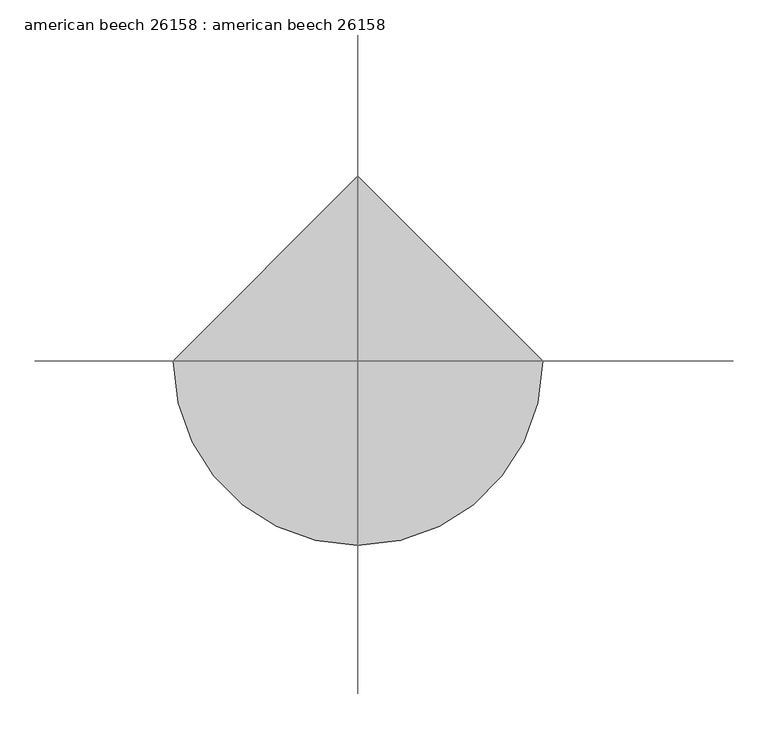
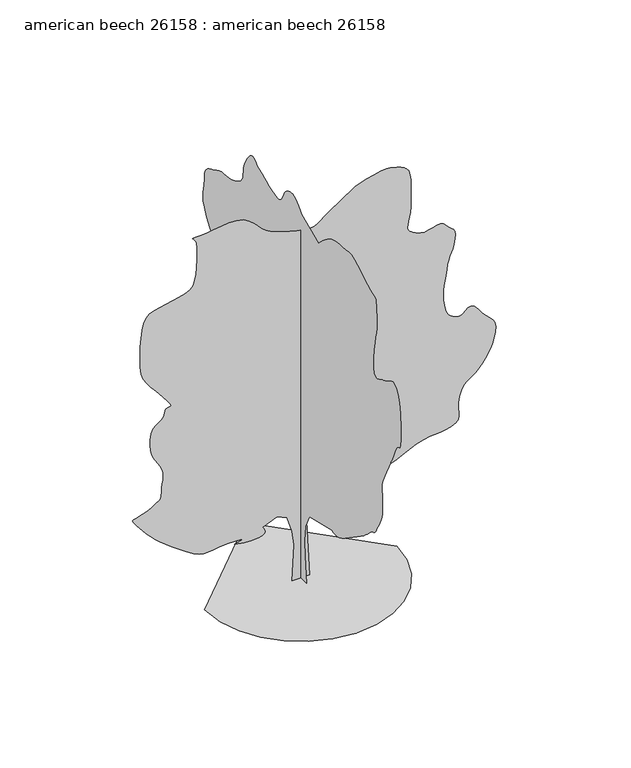
"""IFC4 building model written with IfcOpenShell, lengths in millimetres: proxy geometry, american beech 26158 : american beech 26158."""

from ifc_helpers import new_model, si_unit, origin, place, context, project, spatial, triangles, source, transform, mapped, element, save


def american_beech_26158_american_beech_26158_b3c041c8(model_context):
    return source(origin(), model_context, "Body", "Tessellation", [
        triangles([(0.0009889, 136.856581, 0.0), (0.0009889, -149.8547884, 0.0), (0.0009889, -111.6264895, 420.510052), (0.0009889, -102.0697236, 659.4353302), (0.0009889, -121.1832463, 898.3606447), (0.0009889, -235.8678885, 1118.172373), (0.0009889, -818.8458761, 1261.5275036), (0.0009889, -849.9431059, 1249.7139805), (0.0009889, -883.2933231, 1240.7427258), (0.0009889, -921.1596891, 1237.4533916), (0.0009889, -965.7976622, 1242.6934788), (0.0009889, -1019.4603024, 1259.3000233), (0.0009889, -1084.4081549, 1290.1152935), (0.0009889, -1162.8992941, 1337.984174), (0.0009889, -1478.2811337, 1557.7959023), (0.0009889, -1522.8632961, 1589.1420994), (0.0009889, -1566.942437, 1618.9819931), (0.0009889, -1611.1893002, 1649.3249084), (0.0009889, -1656.2718681, 1682.1772636), (0.0009889, -1702.8579781, 1719.5406807), (0.0009889, -1751.6183739, 1763.4243393), (0.0009889, -1803.2210381, 1815.834803), (0.0009889, -1847.9404015, 1858.0191467), (0.0009889, -1878.9512993, 1877.1351311), (0.0009889, -1901.2702858, 1884.0440117), (0.0009889, -1919.9112991, 1889.616782), (0.0009889, -1939.8884228, 1904.7196392), (0.0009889, -1966.2180656, 1940.2161644), (0.0009889, -2003.916782, 2006.9774963), (0.0009889, -2044.9607883, 2083.2080177), (0.0009889, -2078.313549, 2145.2324295), (0.0009889, -2104.4754696, 2201.0692829), (0.0009889, -2123.9521877, 2258.7475937), (0.0009889, -2137.244109, 2326.2862038), (0.0009889, -2144.8488773, 2411.7141289), (0.0009889, -2147.2746014, 2523.0550072), (0.0009889, -2142.5373905, 2624.8889076), (0.0009889, -2132.7863869, 2688.2873634), (0.0009889, -2124.7040314, 2730.9338882), (0.0009889, -2124.9835201, 2770.583503), (0.0009889, -2140.3072941, 2824.9394875), (0.0009889, -2177.3659332, 2911.7568626), (0.0009889, -2242.84464, 3048.6883301), (0.0009889, -2308.7119858, 3181.9621719), (0.0009889, -2348.5011269, 3259.3812836), (0.0009889, -2371.2366577, 3301.215358), (0.0009889, -2385.9484051, 3327.6567673), (0.0009889, -2401.6632889, 3358.9496246), (0.0009889, -2427.4088104, 3415.3121727), (0.0009889, -2472.2118896, 3516.9885246), (0.0009889, -2522.8114174, 3609.6476944), (0.0009889, -2561.0332123, 3645.1568642), (0.0009889, -2588.5669968, 3652.9040657), (0.0009889, -2607.0580193, 3662.3273277), (0.0009889, -2618.2087921, 3702.8402618), (0.0009889, -2623.669796, 3803.856189), (0.0009889, -2625.117382, 3994.8390083), (0.0009889, -2615.3639076, 4210.713913), (0.0009889, -2589.2271309, 4371.4450905), (0.0009889, -2551.406765, 4483.8402649), (0.0009889, -2506.5400269, 4554.7824463), (0.0009889, -2459.3391289, 4591.1043571), (0.0009889, -2414.4802391, 4599.6895889), (0.0009889, -2376.641851, 4587.3705734), (0.0009889, -2343.8477772, 4566.9491455), (0.0009889, -2310.8862717, 4546.8576393), (0.0009889, -2277.5893215, 4527.4521378), (0.0009889, -2243.7921112, 4509.0116936), (0.0009889, -2209.3243023, 4491.9426773), (0.0009889, -2174.0232594, 4476.5250137), (0.0009889, -2137.7164639, 4463.1392029), (0.0009889, -2096.4236355, 4443.6572525), (0.0009889, -2049.6139927, 4418.4858238), (0.0009889, -2002.3013283, 4400.6805153), (0.0009889, -1959.504958, 4403.2713455), (0.0009889, -1926.2359131, 4439.313913), (0.0009889, -1907.5110386, 4521.8132378), (0.0009889, -1908.3467434, 4663.8246277), (0.0009889, -1923.6450829, 4819.4253044), (0.0009889, -1942.954224, 4940.7356323), (0.0009889, -1963.266647, 5037.9669067), (0.0009889, -1981.572361, 5121.3298416), (0.0009889, -1994.8642822, 5201.0354416), (0.0009889, -2000.1296585, 5287.2429703), (0.0009889, -1994.3614059, 5390.1634323), (0.0009889, -1986.3653824, 5488.9190323), (0.0009889, -1983.048143, 5559.911792), (0.0009889, -1978.5625156, 5609.3407516), (0.0009889, -1967.0562412, 5643.3764648), (0.0009889, -1942.6748806, 5668.2429703), (0.0009889, -1899.5709709, 5690.0869858), (0.0009889, -1831.8926891, 5715.1063889), (0.0009889, -1748.4408062, 5751.9616974), (0.0009889, -1662.820015, 5800.5261749), (0.0009889, -1576.3582867, 5853.7903656), (0.0009889, -1490.4020508, 5904.6919098), (0.0009889, -1406.2848015, 5946.2207703), (0.0009889, -1325.3426491, 5971.3924896), (0.0009889, -1248.913884, 5973.1447083), (0.0009889, -1174.2403896, 5963.3406555), (0.0009889, -1098.5636135, 5956.711409), (0.0009889, -1023.222064, 5950.5641098), (0.0009889, -949.5518515, 5942.2588028), (0.0009889, -878.8914843, 5929.1264648), (0.0009889, -812.5771454, 5908.4509827), (0.0009889, -751.9472706, 5877.5644958), (0.0009889, -697.9494038, 5841.2678741), (0.0009889, -649.9687569, 5805.9618896), (0.0009889, -607.0045916, 5771.4942261), (0.0009889, -568.0511189, 5737.7119858), (0.0009889, -532.1075644, 5704.4128555), (0.0009889, -498.1706097, 5671.4433563), (0.0009889, -465.2369368, 5638.6523346), (0.0009889, -16.056217, 5829.7871796), (0.0009889, 22.8405617, 5872.4339951), (0.0009889, 61.6537222, 5913.023378), (0.0009889, 100.2998553, 5949.3961578), (0.0009889, 138.6950317, 5979.5204819), (0.0009889, 176.7559443, 6001.2883392), (0.0009889, 214.3990318, 6012.5911377), (0.0009889, 251.5404602, 6011.3720261), (0.0009889, 287.2056524, 6002.4312927), (0.0009889, 320.3628219, 5991.305809), (0.0009889, 350.8454089, 5977.0055191), (0.0009889, 378.4856913, 5958.5397858), (0.0009889, 403.1160919, 5934.892392), (0.0009889, 424.5689612, 5905.047702), (0.0009889, 442.6817001, 5868.0144974), (0.0009889, 459.9562634, 5826.9425858), (0.0009889, 480.2407084, 5787.547316), (0.0009889, 505.3740581, 5752.6727005), (0.0009889, 537.1926464, 5725.138916), (0.0009889, 577.5380399, 5707.7911377), (0.0009889, 628.2491524, 5703.5239563), (0.0009889, 691.1650068, 5715.1063889), (0.0009889, 759.6790661, 5736.9754028), (0.0009889, 826.1890326, 5761.3593796), (0.0009889, 891.0251186, 5787.8263687), (0.0009889, 954.5251671, 5815.9694183), (0.0009889, 1017.0218611, 5845.3577408), (0.0009889, 1078.8506453, 5875.5832214), (0.0009889, 1140.3440575, 5906.2412338), (0.0009889, 1169.0715191, 5932.3524307), (0.0009889, 1198.1316639, 5955.3649796), (0.0009889, 1227.8624073, 5972.2052307), (0.0009889, 1258.5938164, 5979.7489563), (0.0009889, 1290.6664227, 5974.9230881), (0.0009889, 1324.4078224, 5954.6539764), (0.0009889, 1360.1557858, 5915.7918137), (0.0009889, 1395.1799561, 5868.217392), (0.0009889, 1426.1908539, 5822.9544571), (0.0009889, 1452.6880737, 5778.8856354), (0.0009889, 1474.1715008, 5734.7912338), (0.0009889, 1490.1379681, 5689.5538788), (0.0009889, 1500.0845993, 5641.9538773), (0.0009889, 1503.510989, 5590.8494385), (0.0009889, 1507.2168674, 5539.3380478), (0.0009889, 1519.1142517, 5491.1793594), (0.0009889, 1540.3740005, 5446.1704788), (0.0009889, 1572.1672634, 5404.1846695), (0.0009889, 1615.6596668, 5365.0428726), (0.0009889, 1672.0274471, 5328.5689362), (0.0009889, 1742.4363762, 5294.5832199), (0.0009889, 1817.5288857, 5269.1836075), (0.0009889, 1887.9378147, 5255.1373718), (0.0009889, 1954.8363476, 5247.4407486), (0.0009889, 2019.3956337, 5241.0911362), (0.0009889, 2082.7839157, 5231.0580276), (0.0009889, 2146.1721977, 5212.3382401), (0.0009889, 2210.7313385, 5179.9024292), (0.0009889, 2276.3498623, 5145.3580261), (0.0009889, 2340.1267834, 5118.8404587), (0.0009889, 2399.0573433, 5093.1356323), (0.0009889, 2450.1315514, 5061.106192), (0.0009889, 2490.3372368, 5015.5136261), (0.0009889, 2516.667025, 4949.193837), (0.0009889, 2526.1132507, 4854.9597633), (0.0009889, 2532.46577, 4758.008123), (0.0009889, 2546.5044479, 4681.9348595), (0.0009889, 2560.7285797, 4617.2411339), (0.0009889, 2567.5865913, 4554.3760757), (0.0009889, 2559.5600464, 4483.8402649), (0.0009889, 2529.1232414, 4396.0578323), (0.0009889, 2468.7702393, 4281.5543564), (0.0009889, 2394.0992157, 4166.6192207), (0.0009889, 2326.6139454, 4078.2525215), (0.0009889, 2267.6553349, 4007.9707649), (0.0009889, 2218.5596397, 3947.1884285), (0.0009889, 2180.6679119, 3887.4223091), (0.0009889, 2155.3111748, 3820.1377533), (0.0009889, 2143.8328056, 3736.8001076), (0.0009889, 2149.4334812, 3646.0204742), (0.0009889, 2171.0820145, 3561.7686401), (0.0009889, 2203.7667927, 3483.5112076), (0.0009889, 2242.4687908, 3410.790937), (0.0009889, 2282.1714546, 3343.1000107), (0.0009889, 2317.8662235, 3279.9047401), (0.0009889, 2344.5311657, 3220.7225967), (0.0009889, 2370.3577869, 3180.6921913), (0.0009889, 2402.5396889, 3164.8934464), (0.0009889, 2434.5538685, 3157.7813805), (0.0009889, 2459.8827003, 3143.8113029), (0.0009889, 2472.0037628, 3107.4638123), (0.0009889, 2464.3963783, 3033.1433487), (0.0009889, 2430.5432121, 2905.3305107), (0.0009889, 2383.9011463, 2761.3378464), (0.0009889, 2340.6017544, 2643.9136185), (0.0009889, 2298.1379219, 2545.7425758), (0.0009889, 2254.0028252, 2459.415287), (0.0009889, 2205.6894951, 2377.6095245), (0.0009889, 2150.6857304, 2292.9614937), (0.0009889, 2086.4897942, 2198.1177189), (0.0009889, 2022.098085, 2102.5196297), (0.0009889, 1968.0723129, 2019.6267242), (0.0009889, 1924.2446102, 1948.102747), (0.0009889, 1890.4447838, 1886.6067913), (0.0009889, 1866.5103436, 1833.8078339), (0.0009889, 1852.2735672, 1788.3620613), (0.0009889, 1847.564407, 1748.9361248), (0.0009889, 1851.5776794, 1721.8800728), (0.0009889, 1860.940044, 1709.2029396), (0.0009889, 1871.6386642, 1703.0459026), (0.0009889, 1879.6624477, 1695.5504299), (0.0009889, 1881.0010288, 1678.8600243), (0.0009889, 1871.6386642, 1645.1186245), (0.0009889, 1847.564407, 1586.4675533), (0.0009889, 1827.5314728, 1524.5828133), (0.0009889, 1825.3850922, 1482.2587978), (0.0009889, 1829.7590984, 1453.3104195), (0.0009889, 1829.2865982, 1431.547649), (0.0009889, 1812.5961926, 1410.7907764), (0.0009889, 1768.3214241, 1384.8497726), (0.0009889, 1685.0958355, 1347.5421661), (0.0009889, 1594.399918, 1309.4244347), (0.0009889, 1528.281134, 1282.5080544), (0.0009889, 1476.2059696, 1262.7823689), (0.0009889, 1427.6412014, 1246.2316349), (0.0009889, 1372.05317, 1228.8453415), (0.0009889, 1298.9138844, 1206.6102161), (0.0009889, 1197.6871416, 1175.5154572), (0.0009889, 1096.069289, 1145.7009253), (0.0009889, 1022.5387482, 1127.7557997), (0.0009889, 967.7331545, 1118.3400227), (0.0009889, 922.2874546, 1114.10329), (0.0009889, 876.8442255, 1111.7080873), (0.0009889, 822.0360884, 1107.806654), (0.0009889, 748.5055475, 1099.0588594), (0.0009889, 662.4935011, 1085.0990284), (0.0009889, 576.4788749, 1068.1292793), (0.0009889, 490.4667558, 1048.6551046), (0.0009889, 404.4521296, 1027.1717503), (0.0009889, 318.4400468, 1004.1847086), (0.0009889, 232.4266923, 980.1943851), (0.0009889, 146.4133378, 955.7037289), (136.1842383, 0.0003154, 0.014068), (-131.4120823, 0.0003154, 0.014068), (-102.7410489, 0.0002819, 563.8778998), (-131.4120823, 0.0002692, 793.2477293), (-207.8684348, 0.0002549, 1032.1729712), (-360.7819027, 0.0002501, 1108.6296415), (-580.5936673, 0.0002549, 1013.0594576), (-562.704425, 0.0002564, 988.5662579), (-548.0765751, 0.000258, 964.5784779), (-539.9688578, 0.0002596, 941.5914362), (-541.6401947, 0.0002612, 920.1080818), (-556.3518694, 0.0002628, 900.6313637), (-587.3627672, 0.0002628, 883.6641581), (-637.9342443, 0.0002644, 869.704327), (-697.421093, 0.0002644, 860.4815615), (-753.4001616, 0.0002644, 856.775683), (-806.4506298, 0.0002644, 857.667271), (-857.1617786, 0.0002644, 862.2366869), (-906.117802, 0.0002644, 869.5645826), (-953.9028214, 0.0002628, 878.731465), (-1001.1011759, 0.0002628, 888.8178406), (-953.2881786, 0.0002628, 900.9945683), (-913.501581, 0.0002612, 912.5008427), (-889.7601522, 0.0002612, 922.6710068), (-890.0954515, 0.0002596, 930.8345346), (-922.5287189, 0.0002596, 936.3235165), (-995.0838833, 0.0002596, 938.4698244), (-1115.7848007, 0.0002596, 936.6028599), (-1242.9524746, 0.0002612, 927.8271601), (-1337.3542706, 0.0002612, 914.3677345), (-1410.6891838, 0.0002612, 903.2500992), (-1474.6617325, 0.0002612, 901.4949738), (-1540.9759987, 0.0002612, 916.12286), (-1621.3340298, 0.0002596, 954.1568756), (-1727.4351116, 0.0002549, 1022.614979), (-1845.0726986, 0.0002501, 1105.8432564), (-1952.34711, 0.0002453, 1184.0549795), (-2049.4209812, 0.0002405, 1258.0858532), (-2136.46436, 0.0002373, 1328.7765965), (-2213.6472942, 0.0002326, 1396.9554291), (-2281.1300938, 0.0002278, 1463.4653229), (-2339.0852772, 0.0002246, 1529.1396572), (-2391.8031349, 0.0002214, 1592.6651402), (-2441.3431343, 0.0002166, 1651.1791557), (-2484.5309052, 0.0002134, 1703.170459), (-2518.1884438, 0.0002118, 1747.1378334), (-2539.1409439, 0.0002103, 1781.577737), (-2544.218541, 0.0002087, 1804.9838665), (-2530.2254997, 0.0002071, 1815.8500637), (-2498.742247, 0.0002071, 1822.7308937), (-2456.2227493, 0.0002071, 1834.628278), (-2406.8475655, 0.0002055, 1850.7065117), (-2354.8003063, 0.0002039, 1870.1272739), (-2304.2568798, 0.0002023, 1892.0551506), (-2259.3978447, 0.0002023, 1915.6542915), (-2224.401725, 0.0002007, 1940.091608), (-2196.9849392, 0.0001991, 1958.6464348), (-2172.4078056, 0.0001991, 1969.1798035), (-2151.1759621, 0.0001975, 1977.7066086), (-2133.7896687, 0.0001975, 1990.2439247), (-2120.7518017, 0.0001959, 2012.8144947), (-2112.5602959, 0.0001927, 2051.4326317), (-2109.7180275, 0.0001895, 2112.118317), (-2105.7607109, 0.0001864, 2181.0514641), (-2096.7894562, 0.0001816, 2242.2935108), (-2087.1476028, 0.0001784, 2298.6891964), (-2081.1861935, 0.0001752, 2353.0781731), (-2083.2487129, 0.000172, 2408.3028545), (-2097.6809715, 0.0001688, 2467.2028931), (-2128.8315411, 0.0001641, 2532.6259346), (-2168.3971493, 0.0001609, 2596.7202782), (-2204.2849297, 0.0001577, 2653.2860115), (-2235.1560104, 0.0001545, 2707.6675758), (-2259.6771881, 0.0001513, 2765.2239464), (-2276.5047947, 0.0001465, 2831.3149704), (-2284.3076614, 0.0001418, 2911.2740433), (-2281.7447365, 0.000137, 3010.4865921), (-2264.5514545, 0.0001306, 3102.7902603), (-2233.1494469, 0.0001274, 3164.9948936), (-2193.2231049, 0.0001242, 3206.8286774), (-2150.4520237, 0.0001226, 3237.9439293), (-2110.525827, 0.0001211, 3268.0682533), (-2079.123674, 0.0001179, 3306.8795471), (-2061.9330082, 0.0001147, 3364.0804161), (-2043.9599773, 0.0001131, 3413.0262657), (-2014.1200836, 0.0001115, 3431.3396828), (-1983.9422745, 0.0001115, 3435.3019409), (-1964.9684326, 0.0001099, 3441.0931572), (-1968.7301216, 0.0001099, 3464.9437363), (-2006.7641373, 0.0001051, 3523.0843735), (-2090.6020432, 9.88e-05, 3631.6948952), (-2191.4121689, 9.24e-05, 3753.7165169), (-2273.3296978, 8.6e-05, 3849.6778107), (-2337.3582024, 8.12e-05, 3932.1009773), (-2384.5031445, 7.65e-05, 4013.5079269), (-2415.7654804, 7.17e-05, 4106.47202), (-2432.1484921, 6.37e-05, 4223.4898773), (-2434.6554611, 5.42e-05, 4377.1345688), (-2429.5297565, 4.46e-05, 4541.5998207), (-2420.5585018, 3.66e-05, 4683.0016548), (-2405.0643894, 3.03e-05, 4801.6705742), (-2380.3781055, 2.39e-05, 4897.9365005), (-2343.822488, 1.91e-05, 4972.1558075), (-2292.720084, 1.59e-05, 5024.6066757), (-2224.401725, 1.43e-05, 5055.6710587), (-2138.4149677, 1.27e-05, 5074.7972168), (-2040.8941761, 1.27e-05, 5092.7292618), (-1939.0274288, 1.11e-05, 5111.8554199), (-1840.0028046, 9.6e-06, 5134.487178), (-1751.0088181, 8e-06, 5162.9604401), (-1679.2334026, 6.4e-06, 5199.612854), (-1631.8649277, 3.2e-06, 5246.8314835), (-1604.1128426, -1.6e-06, 5316.4272354), (-1585.3905842, -6.4e-06, 5411.6010773), (-1574.1890877, -1.27e-05, 5521.6594757), (-1569.0075726, -2.07e-05, 5635.9088974), (-1568.336974, -2.71e-05, 5743.6302292), (-1570.6788368, -3.19e-05, 5834.1305191), (-1574.524387, -3.5e-05, 5896.690654), (-1585.918895, -3.82e-05, 5936.1626633), (-1606.0102558, -3.98e-05, 5965.4230865), (-1625.9315689, -4.14e-05, 5985.9718323), (-1636.825526, -4.14e-05, 5999.3576431), (-1629.8329296, -4.3e-05, 6007.0286865), (-1596.0890591, -4.3e-05, 6010.559285), (-1526.7393677, -4.3e-05, 6011.3976059), (-1428.7715103, -4.3e-05, 6017.8233765), (-1318.7690678, -4.46e-05, 6032.4538788), (-1202.2439129, -4.46e-05, 6048.2529144), (-1084.7180197, -4.46e-05, 6058.184285), (-971.7057318, -4.46e-05, 6055.263533), (-868.7238636, -4.46e-05, 6032.4538788), (-781.2893749, -4.14e-05, 5982.7208679), (-714.8937183, -3.66e-05, 5922.6245361), (-665.5465851, -3.34e-05, 5871.6974121), (-624.5610781, -3.19e-05, 5827.4756927), (-583.2403444, -2.87e-05, 5787.445578), (-532.8924365, -2.71e-05, 5749.0915237), (-464.8228995, -2.39e-05, 5709.8735687), (-370.3373878, -2.23e-05, 5667.3284912), (-260.8632923, -1.91e-05, 5627.3745346), (-155.7366604, -1.75e-05, 5596.9449966), (-58.1322665, -1.59e-05, 5575.0504028), (28.7726351, -1.59e-05, 5560.6739548), (101.8020074, -1.59e-05, 5552.8255966), (157.7788323, -1.43e-05, 5550.4629501), (193.5270681, -1.59e-05, 5552.6477005), (219.2725352, -1.59e-05, 5560.6233765), (247.3583572, -1.59e-05, 5575.4311935), (277.7847885, -1.75e-05, 5595.7770447), (310.5508118, -1.91e-05, 5620.2877579), (345.6587342, -2.07e-05, 5647.6692261), (383.1059761, -2.23e-05, 5676.5232788), (422.8950809, -2.39e-05, 5705.555809), (805.1781057, -3.98e-05, 5963.5947098), (830.3647951, -3.98e-05, 5972.992392), (896.679134, -4.14e-05, 5996.5892075), (990.2426817, -4.3e-05, 6027.5518524), (1097.1817938, -4.62e-05, 6058.9970261), (1203.6180296, -4.62e-05, 6084.1175858), (1295.67789, -4.78e-05, 6096.0046509), (1359.4853325, -4.78e-05, 6087.8516602), (1407.4912685, -4.62e-05, 6070.6556168), (1459.1777939, -4.46e-05, 6056.8128571), (1511.1996185, -4.46e-05, 6041.4457718), (1560.2089817, -4.3e-05, 6019.7540726), (1602.8682964, -4.14e-05, 5986.835733), (1635.8299473, -3.82e-05, 5937.8898834), (1655.7537312, -3.34e-05, 5868.0394958), (1665.3091072, -2.87e-05, 5789.7820633), (1670.1859898, -2.55e-05, 5717.2399796), (1671.5500053, -2.07e-05, 5647.8471222), (1670.5746288, -1.75e-05, 5579.1396881), (1668.4282482, -1.27e-05, 5508.6038773), (1666.2844837, -8e-06, 5433.699147), (1665.3091072, -3.2e-06, 5351.9622757), (1660.2367424, 1.6e-06, 5270.5806152), (1648.1463467, 6.4e-06, 5198.4187408), (1633.7114719, 9.6e-06, 5135.2743393), (1621.6186054, 1.27e-05, 5081.0200928), (1616.5487114, 1.59e-05, 5035.4269455), (1623.1807194, 1.75e-05, 4998.368161), (1646.1955936, 1.91e-05, 4969.6664246), (1678.4054008, 2.07e-05, 4946.8317719), (1709.6119263, 2.23e-05, 4927.324823), (1739.9826015, 2.23e-05, 4910.992099), (1769.6829689, 2.39e-05, 4897.6824463), (1798.8852562, 2.39e-05, 4887.1923889), (1827.7499187, 2.55e-05, 4879.3946091), (1856.4493298, 2.55e-05, 4874.0862122), (1893.0609032, 2.55e-05, 4877.1087021), (1942.2125542, 2.39e-05, 4889.9864044), (1998.8851124, 2.39e-05, 4906.1918106), (2058.0671104, 2.23e-05, 4919.2474091), (2114.7396687, 2.23e-05, 4922.5745316), (2163.8911743, 2.39e-05, 4909.6968292), (2200.5028931, 2.55e-05, 4874.0862122), (2230.4850746, 2.71e-05, 4834.208123), (2261.3003448, 2.87e-05, 4807.6649757), (2290.2766285, 3.03e-05, 4786.8368866), (2314.7419956, 3.19e-05, 4763.9769447), (2332.0165226, 3.34e-05, 4731.4396866), (2339.4282795, 3.66e-05, 4681.5031998), (2334.3025749, 4.14e-05, 4606.4970222), (2319.8956055, 4.62e-05, 4526.9440292), (2302.1485783, 4.94e-05, 4463.951944), (2282.3925167, 5.26e-05, 4410.6627548), (2261.9683273, 5.57e-05, 4360.1928703), (2242.2147366, 5.89e-05, 4305.7098587), (2224.4652386, 6.37e-05, 4240.3809975), (2210.0608852, 6.85e-05, 4157.3229858), (2196.9087811, 7.33e-05, 4068.4481781), (2183.2562714, 7.8e-05, 3988.0827347), (2170.9397266, 8.28e-05, 3913.0762665), (2161.8007496, 8.76e-05, 3840.2289688), (2157.6783268, 9.08e-05, 3766.3913246), (2160.4088287, 9.56e-05, 3688.3876556), (2171.831242, 0.0001003, 3603.0181572), (2189.9719952, 0.0001051, 3525.0147789), (2211.6203831, 0.0001083, 3468.2711494), (2236.7791672, 0.0001115, 3428.240744), (2265.4506729, 0.0001131, 3400.402327), (2297.6324295, 0.0001147, 3380.2602425), (2333.3271984, 0.0001147, 3363.2673843), (2372.5296021, 0.0001163, 3344.9795471), (2412.5675652, 0.0001163, 3342.4901642), (2451.7724396, 0.0001147, 3366.0869797), (2491.642971, 0.0001131, 3400.8848557), (2533.6901138, 0.0001115, 3432.0253967), (2579.4227875, 0.0001099, 3444.5728867), (2630.3246223, 0.0001115, 3423.7195084), (2687.906282, 0.0001163, 3354.5298363), (2749.8568611, 0.0001211, 3269.9730789), (2810.1313797, 0.0001242, 3206.9557045), (2864.6905495, 0.0001274, 3156.6637161), (2909.5976921, 0.0001306, 3110.2325386), (2940.7635223, 0.0001338, 3058.7720169), (2954.2254913, 0.000137, 2993.4178665), (2945.9451828, 0.0001434, 2905.3557999), (2924.1520363, 0.0001481, 2810.6139084), (2899.209082, 0.0001529, 2729.079641), (2870.2277115, 0.0001577, 2657.6040619), (2836.3948929, 0.0001609, 2592.9612053), (2796.8723053, 0.0001641, 2531.9858574), (2750.8474983, 0.0001688, 2471.5235596), (2697.4568619, 0.000172, 2408.3842449), (2642.4404526, 0.0001752, 2354.2186558), (2591.9196991, 0.0001784, 2316.7713776), (2545.7425758, 0.00018, 2287.0127289), (2503.7637428, 0.0001816, 2255.9181152), (2465.7858284, 0.0001832, 2214.4575645), (2431.6531734, 0.000188, 2153.606773), (2401.2011078, 0.0001927, 2064.3332977), (2384.7901909, 0.0001991, 1965.7532684), (2385.7654221, 0.0002039, 1881.8849865), (2393.4261463, 0.0002071, 1811.0570423), (2397.0760689, 0.0002118, 1751.5981716), (2386.0143894, 0.000215, 1701.8343487), (2349.5424877, 0.0002166, 1660.0945999), (2276.9594181, 0.0002182, 1624.7096958), (2189.7484623, 0.0002198, 1601.1638947), (2111.7322941, 0.0002214, 1590.8261536), (2035.7202187, 0.0002214, 1585.8401207), (1954.5264828, 0.0002214, 1578.3445026), (1860.9630077, 0.000223, 1560.4858543), (1747.8389534, 0.0002246, 1524.4025917), (1607.9660957, 0.0002294, 1462.2385082), (1455.667543, 0.0002326, 1390.7425816), (1311.7282185, 0.0002357, 1331.4512878), (1178.6524023, 0.0002389, 1283.6941738), (1058.9547667, 0.0002421, 1246.8031116), (955.1372663, 0.0002437, 1220.1102642), (869.7094139, 0.0002437, 1202.9449602), (805.1781057, 0.0002453, 1194.641688), (403.7815673, 0.0002453, 1185.0862392), (107.513205, 0.0002485, 1137.3011473), (88.3996914, 0.0002628, 879.2597757), (-1453.7574852, 0.0, 0.0120292), (-1415.3246567, -333.1060121, 0.0120292), (-1305.8708725, -639.0085974, 0.0120292), (-1134.1566444, -908.9473532, 0.0120292), (-908.9473532, -1134.1566444, 0.0120292), (-639.0085974, -1305.8708725, 0.0120292), (-333.1060121, -1415.3246567, 0.0120292), (6.35e-05, -1453.7574852, 0.0120292), (333.1060121, -1415.3246567, 0.0120292), (639.0085974, -1305.8708725, 0.0120292), (908.9473532, -1134.1566444, 0.0120292), (1134.1566444, -908.9473532, 0.0120292), (1305.8708725, -639.0085974, 0.0120292), (1415.3246567, -333.1060121, 0.0120292), (1453.7574852, 0.0001274, 0.0120292), (-0.0001906, 1453.7574852, 0.0120292)], [[1, 2, 3], [254, 1, 3], [254, 3, 4], [254, 4, 5], [254, 5, 6], [53, 54, 55], [52, 53, 55], [201, 202, 203], [201, 203, 204], [200, 201, 204], [222, 223, 224], [52, 55, 56], [200, 204, 205], [199, 200, 205], [253, 254, 6], [221, 222, 224], [221, 224, 225], [229, 230, 231], [229, 231, 232], [228, 229, 232], [228, 232, 233], [227, 228, 233], [252, 253, 6], [221, 225, 226], [220, 221, 226], [199, 205, 206], [198, 199, 206], [62, 63, 64], [61, 62, 64], [61, 64, 65], [60, 61, 65], [60, 65, 66], [59, 60, 66], [59, 66, 67], [59, 67, 68], [58, 59, 68], [58, 68, 69], [58, 69, 70], [57, 58, 70], [57, 70, 71], [57, 71, 72], [57, 72, 73], [57, 73, 74], [56, 57, 74], [52, 56, 74], [51, 52, 74], [50, 51, 74], [50, 74, 75], [49, 50, 75], [48, 49, 75], [47, 48, 75], [46, 47, 75], [45, 46, 75], [44, 45, 75], [43, 44, 75], [42, 43, 75], [42, 75, 76], [41, 42, 76], [227, 233, 234], [226, 227, 234], [220, 226, 234], [219, 220, 234], [219, 234, 235], [219, 235, 236], [219, 236, 237], [218, 219, 237], [218, 237, 238], [218, 238, 239], [218, 239, 240], [217, 218, 240], [217, 240, 241], [217, 241, 242], [217, 242, 243], [217, 243, 244], [217, 244, 245], [217, 245, 246], [216, 217, 246], [216, 246, 247], [215, 216, 247], [215, 247, 248], [251, 252, 6], [88, 89, 90], [88, 90, 91], [87, 88, 91], [87, 91, 92], [86, 87, 92], [86, 92, 93], [85, 86, 93], [84, 85, 93], [84, 93, 94], [83, 84, 94], [82, 83, 94], [81, 82, 94], [81, 94, 95], [80, 81, 95], [80, 95, 96], [80, 96, 97], [80, 97, 98], [80, 98, 99], [80, 99, 100], [80, 100, 101], [80, 101, 102], [80, 102, 103], [80, 103, 104], [80, 104, 105], [80, 105, 106], [80, 106, 107], [80, 107, 108], [80, 108, 109], [80, 109, 110], [80, 110, 111], [80, 111, 112], [79, 80, 112], [79, 112, 113], [78, 79, 113], [77, 78, 113], [76, 77, 113], [41, 76, 113], [40, 41, 113], [40, 113, 114], [39, 40, 114], [198, 206, 207], [197, 198, 207], [196, 197, 207], [196, 207, 208], [195, 196, 208], [195, 208, 209], [195, 209, 210], [195, 210, 211], [194, 195, 211], [194, 211, 212], [194, 212, 213], [193, 194, 213], [193, 213, 214], [214, 215, 248], [193, 214, 248], [193, 248, 249], [192, 193, 249], [192, 249, 250], [192, 250, 251], [192, 251, 6], [192, 6, 7], [191, 192, 7], [190, 191, 7], [189, 190, 7], [38, 39, 114], [37, 38, 114], [36, 37, 114], [35, 36, 114], [34, 35, 114], [33, 34, 114], [32, 33, 114], [31, 32, 114], [30, 31, 114], [29, 30, 114], [28, 29, 114], [27, 28, 114], [26, 27, 114], [25, 26, 114], [24, 25, 114], [23, 24, 114], [22, 23, 114], [21, 22, 114], [20, 21, 114], [19, 20, 114], [18, 19, 114], [17, 18, 114], [16, 17, 114], [15, 16, 114], [14, 15, 114], [13, 14, 114], [12, 13, 114], [11, 12, 114], [10, 11, 114], [9, 10, 114], [8, 9, 114], [7, 8, 114], [189, 7, 114], [188, 189, 114], [188, 114, 115], [188, 115, 116], [188, 116, 117], [188, 117, 118], [188, 118, 119], [188, 119, 120], [188, 120, 121], [146, 147, 148], [145, 146, 148], [144, 145, 148], [144, 148, 149], [143, 144, 149], [143, 149, 150], [142, 143, 150], [142, 150, 151], [142, 151, 152], [141, 142, 152], [141, 152, 153], [141, 153, 154], [141, 154, 155], [141, 155, 156], [140, 141, 156], [140, 156, 157], [139, 140, 157], [138, 139, 157], [138, 157, 158], [137, 138, 158], [137, 158, 159], [136, 137, 159], [135, 136, 159], [135, 159, 160], [134, 135, 160], [134, 160, 161], [174, 175, 176], [173, 174, 176], [173, 176, 177], [172, 173, 177], [171, 172, 177], [171, 177, 178], [170, 171, 178], [170, 178, 179], [169, 170, 179], [168, 169, 179], [167, 168, 179], [166, 167, 179], [165, 166, 179], [165, 179, 180], [165, 180, 181], [165, 181, 182], [165, 182, 183], [165, 183, 184], [165, 184, 185], [165, 185, 186], [165, 186, 187], [164, 165, 187], [164, 187, 188], [163, 164, 188], [162, 163, 188], [161, 162, 188], [134, 161, 188], [133, 134, 188], [132, 133, 188], [125, 126, 127], [124, 125, 127], [124, 127, 128], [123, 124, 128], [122, 123, 128], [121, 122, 128], [121, 128, 129], [121, 129, 130], [121, 130, 131], [188, 121, 131], [132, 188, 131], [274, 275, 276], [531, 255, 256], [531, 256, 257], [531, 257, 258], [531, 258, 259], [530, 531, 259], [376, 377, 378], [376, 378, 379], [375, 376, 379], [273, 274, 276], [273, 276, 277], [375, 379, 380], [374, 375, 380], [273, 277, 278], [272, 273, 278], [301, 302, 303], [301, 303, 304], [300, 301, 304], [300, 304, 305], [299, 300, 305], [299, 305, 306], [298, 299, 306], [298, 306, 307], [297, 298, 307], [297, 307, 308], [271, 272, 278], [296, 297, 308], [296, 308, 309], [373, 374, 380], [373, 380, 381], [372, 373, 381], [295, 296, 309], [295, 309, 310], [294, 295, 310], [294, 310, 311], [294, 311, 312], [294, 312, 313], [293, 294, 313], [293, 313, 314], [292, 293, 314], [271, 278, 279], [291, 292, 314], [530, 259, 260], [372, 381, 382], [371, 372, 382], [291, 314, 315], [290, 291, 315], [371, 382, 383], [370, 371, 383], [370, 383, 384], [369, 370, 384], [369, 384, 385], [369, 385, 386], [369, 386, 387], [369, 387, 388], [369, 388, 389], [369, 389, 390], [368, 369, 390], [368, 390, 391], [367, 368, 391], [367, 391, 392], [367, 392, 393], [366, 367, 393], [366, 393, 394], [270, 271, 279], [366, 394, 395], [338, 339, 340], [338, 340, 341], [289, 290, 315], [483, 484, 485], [483, 485, 486], [482, 483, 486], [481, 482, 486], [481, 486, 487], [480, 481, 487], [288, 289, 315], [287, 288, 315], [286, 287, 315], [285, 286, 315], [284, 285, 315], [283, 284, 315], [282, 283, 315], [282, 315, 316], [281, 282, 316], [281, 316, 317], [281, 317, 318], [281, 318, 319], [281, 319, 320], [280, 281, 320], [280, 320, 321], [279, 280, 321], [279, 321, 322], [480, 487, 488], [264, 265, 266], [263, 264, 266], [263, 266, 267], [262, 263, 267], [262, 267, 268], [261, 262, 268], [261, 268, 269], [261, 269, 270], [261, 270, 279], [261, 279, 322], [260, 261, 322], [530, 260, 322], [530, 322, 323], [529, 530, 323], [529, 323, 324], [366, 395, 396], [365, 366, 396], [337, 338, 341], [337, 341, 342], [529, 324, 325], [528, 529, 325], [527, 528, 325], [526, 527, 325], [525, 526, 325], [524, 525, 325], [523, 524, 325], [522, 523, 325], [521, 522, 325], [521, 325, 326], [521, 326, 327], [521, 327, 328], [521, 328, 329], [521, 329, 330], [521, 330, 331], [521, 331, 332], [521, 332, 333], [521, 333, 334], [521, 334, 335], [521, 335, 336], [521, 336, 337], [521, 337, 342], [520, 521, 342], [520, 342, 343], [519, 520, 343], [518, 519, 343], [518, 343, 344], [517, 518, 344], [449, 450, 451], [448, 449, 451], [448, 451, 452], [447, 448, 452], [446, 447, 452], [446, 452, 453], [516, 517, 344], [515, 516, 344], [514, 515, 344], [513, 514, 344], [512, 513, 344], [511, 512, 344], [510, 511, 344], [509, 510, 344], [508, 509, 344], [507, 508, 344], [506, 507, 344], [505, 506, 344], [504, 505, 344], [503, 504, 344], [502, 503, 344], [501, 502, 344], [500, 501, 344], [499, 500, 344], [498, 499, 344], [497, 498, 344], [496, 497, 344], [495, 496, 344], [494, 495, 344], [493, 494, 344], [492, 493, 344], [491, 492, 344], [490, 491, 344], [489, 490, 344], [488, 489, 344], [480, 488, 344], [479, 480, 344], [478, 479, 344], [477, 478, 344], [476, 477, 344], [475, 476, 344], [474, 475, 344], [473, 474, 344], [472, 473, 344], [471, 472, 344], [470, 471, 344], [469, 470, 344], [468, 469, 344], [467, 468, 344], [466, 467, 344], [465, 466, 344], [464, 465, 344], [463, 464, 344], [463, 344, 345], [462, 463, 345], [462, 345, 346], [461, 462, 346], [460, 461, 346], [459, 460, 346], [458, 459, 346], [457, 458, 346], [456, 457, 346], [455, 456, 346], [454, 455, 346], [453, 454, 346], [446, 453, 346], [445, 446, 346], [444, 445, 346], [443, 444, 346], [442, 443, 346], [441, 442, 346], [440, 441, 346], [439, 440, 346], [438, 439, 346], [437, 438, 346], [436, 437, 346], [435, 436, 346], [435, 346, 347], [435, 347, 348], [435, 348, 349], [435, 349, 350], [435, 350, 351], [435, 351, 352], [435, 352, 353], [435, 353, 354], [435, 354, 355], [435, 355, 356], [435, 356, 357], [435, 357, 358], [435, 358, 359], [435, 359, 360], [435, 360, 361], [435, 361, 362], [435, 362, 363], [435, 363, 364], [435, 364, 365], [435, 365, 396], [435, 396, 397], [435, 397, 398], [435, 398, 399], [435, 399, 400], [435, 400, 401], [435, 401, 402], [435, 402, 403], [435, 403, 404], [435, 404, 405], [435, 405, 406], [435, 406, 407], [435, 407, 408], [435, 408, 409], [434, 435, 409], [433, 434, 409], [432, 433, 409], [431, 432, 409], [430, 431, 409], [429, 430, 409], [429, 409, 410], [429, 410, 411], [429, 411, 412], [428, 429, 412], [428, 412, 413], [427, 428, 413], [426, 427, 413], [426, 413, 414], [425, 426, 414], [425, 414, 415], [425, 415, 416], [425, 416, 417], [424, 425, 417], [424, 417, 418], [423, 424, 418], [423, 418, 419], [422, 423, 419], [422, 419, 420], [421, 422, 420], [546, 547, 532], [545, 546, 532], [545, 532, 533], [544, 545, 533], [544, 533, 534], [544, 534, 535], [543, 544, 535], [542, 543, 535], [542, 535, 536], [542, 536, 537], [542, 537, 538], [542, 538, 539], [542, 539, 540], [542, 540, 541]], closed=False),
    ])


if __name__ == "__main__":
    model = new_model("IFC4")
    model_context = context("Model", 3, world=origin())
    ifc_project = project(units=[si_unit("LENGTHUNIT", "METRE", prefix="MILLI")], contexts=[model_context])
    site = spatial("IfcSite", under=ifc_project)
    building = spatial("IfcBuilding", under=site)
    placement = place(None, origin())
    american_beech_26158_american_beech_26158_shape = american_beech_26158_american_beech_26158_b3c041c8(model_context)
    element("IfcBuildingElementProxy", 1, Name="american beech 26158 : american beech 26158", ObjectType="american beech 26158 : american beech 26158", at=placement, inside=building, context=model_context, shape_type="MappedRepresentation", body=[
        mapped(american_beech_26158_american_beech_26158_shape, transform((0.0, 0.0, 0.0), x_axis=(1.0, 0.0, 0.0), y_axis=(0.0, 1.0, 0.0), z_axis=(0.0, 0.0, 1.0))),
    ])
    save(model, "model.ifc")

# Revit data of these elements
# Type "american beech 26158 : american beech 26158"
#   built-in parameter 1005195 = "RPC-16-G1GQ-43Q0-7NP3-0000-ST1L-LVER-AU"
#   Height = 0
